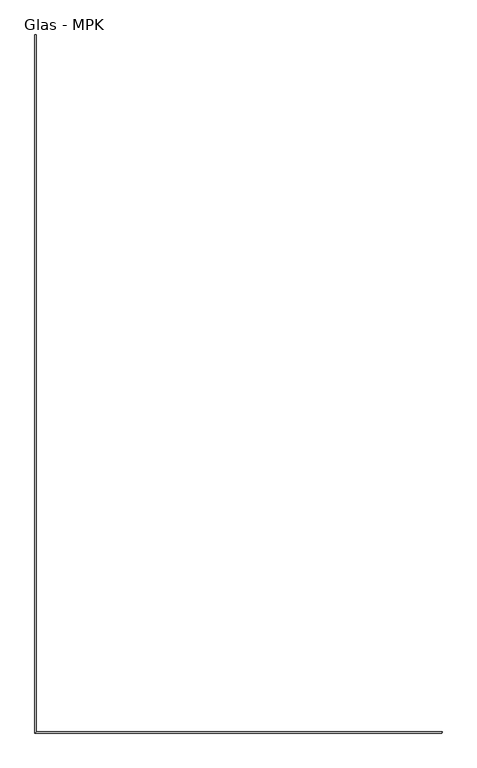
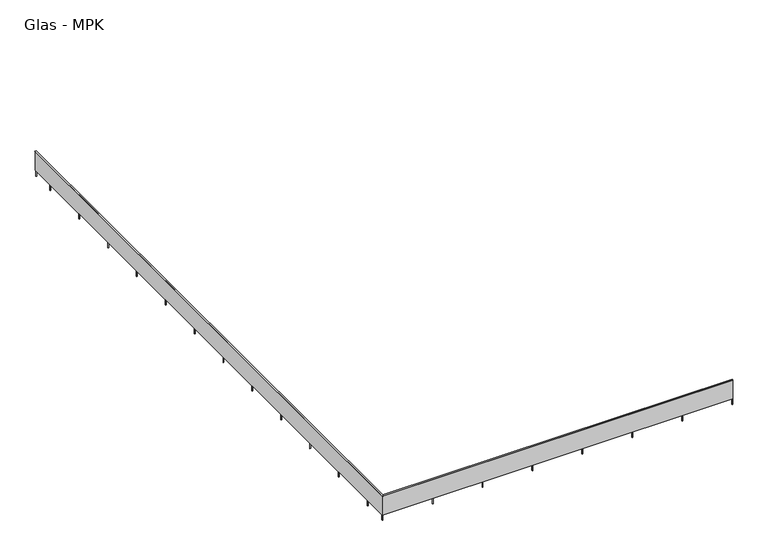
"""IFC4 building model written with IfcOpenShell, lengths in millimetres: railing geometry, Glas - MPK."""

from ifc_helpers import new_model, si_unit, frame, origin, place, context, project, spatial, polyline, outline, extrude, faceted_brep, source, transform, mapped, element, save


def glas_mpk_99f97afc(model_context):
    return source(origin(), model_context, "Body", "SolidModel", [
        faceted_brep([(22257.9971367, 15998.757723, 3843.2628643), (22207.9971367, 15998.757723, 3843.2628643), (22207.9971367, 15998.757723, 3856.7371357), (22257.9971367, 15998.757723, 3856.7371357), (36243.4971367, -8011.242277, 3843.2628643), (36243.4971367, -8011.242277, 3856.7371357), (36243.4971367, -8061.242277, 3856.7371357), (36243.4971367, -8061.242277, 3843.2628643), (22257.9971367, -8011.242277, 3843.2628643), (22207.9971367, -8061.242277, 3843.2628643), (22207.9971367, -8061.242277, 3856.7371357), (22257.9971367, -8011.242277, 3856.7371357)], [[[0, 1, 2, 3]], [[4, 5, 6, 7]], [[1, 0, 8, 9]], [[2, 1, 9, 10]], [[3, 2, 10, 11]], [[0, 3, 11, 8]], [[9, 8, 4, 7]], [[10, 9, 7, 6]], [[11, 10, 6, 5]], [[8, 11, 5, 4]]]),
        faceted_brep([(22217.9971367, 15998.757723, 3842.8769824), (22232.1892606, 15998.757723, 3842.8769824), (22232.1892606, 15998.757723, 3042.8769824), (22217.9971367, 15998.757723, 3042.8769824), (22217.9971367, -8051.242277, 3842.8769824), (22232.1892606, -8037.0501531, 3842.8769824), (22232.1892606, -8037.0501531, 3042.8769824), (22217.9971367, -8051.242277, 3042.8769824), (36243.4971367, -8051.242277, 3842.8769824), (36243.4971367, -8051.242277, 3042.8769824), (36243.4971367, -8037.0501531, 3042.8769824), (36243.4971367, -8037.0501531, 3842.8769824)], [[[0, 1, 2, 3]], [[1, 0, 4, 5]], [[2, 1, 5, 6]], [[3, 2, 6, 7]], [[0, 3, 7, 4]], [[8, 9, 10, 11]], [[5, 4, 8, 11]], [[6, 5, 11, 10]], [[7, 6, 10, 9]], [[4, 7, 9, 8]]]),
        extrude(outline(polyline([(34236.9971367, -8036.242277), (34236.9971367, -8011.242277), (34261.9971367, -8011.242277), (34261.9971367, -8036.242277), (34236.9971367, -8036.242277)])), frame((0.0, 0.0, 2800.0), z_axis=(0.0, 0.0, 1.0), x_axis=(1.0, 0.0, 0.0)), (0.0, 0.0, 1.0), 1043.2628643),
        extrude(outline(polyline([(32236.9971367, -8036.242277), (32236.9971367, -8011.242277), (32261.9971367, -8011.242277), (32261.9971367, -8036.242277), (32236.9971367, -8036.242277)])), frame((0.0, 0.0, 2800.0), z_axis=(0.0, 0.0, 1.0), x_axis=(1.0, 0.0, 0.0)), (0.0, 0.0, 1.0), 1043.2628643),
        extrude(outline(polyline([(30236.9971367, -8036.242277), (30236.9971367, -8011.242277), (30261.9971367, -8011.242277), (30261.9971367, -8036.242277), (30236.9971367, -8036.242277)])), frame((0.0, 0.0, 2800.0), z_axis=(0.0, 0.0, 1.0), x_axis=(1.0, 0.0, 0.0)), (0.0, 0.0, 1.0), 1043.2628643),
        extrude(outline(polyline([(28236.9971367, -8036.242277), (28236.9971367, -8011.242277), (28261.9971367, -8011.242277), (28261.9971367, -8036.242277), (28236.9971367, -8036.242277)])), frame((0.0, 0.0, 2800.0), z_axis=(0.0, 0.0, 1.0), x_axis=(1.0, 0.0, 0.0)), (0.0, 0.0, 1.0), 1043.2628643),
        extrude(outline(polyline([(26236.9971367, -8036.242277), (26236.9971367, -8011.242277), (26261.9971367, -8011.242277), (26261.9971367, -8036.242277), (26236.9971367, -8036.242277)])), frame((0.0, 0.0, 2800.0), z_axis=(0.0, 0.0, 1.0), x_axis=(1.0, 0.0, 0.0)), (0.0, 0.0, 1.0), 1043.2628643),
        extrude(outline(polyline([(24236.9971367, -8036.242277), (24236.9971367, -8011.242277), (24261.9971367, -8011.242277), (24261.9971367, -8036.242277), (24236.9971367, -8036.242277)])), frame((0.0, 0.0, 2800.0), z_axis=(0.0, 0.0, 1.0), x_axis=(1.0, 0.0, 0.0)), (0.0, 0.0, 1.0), 1043.2628643),
        extrude(outline(polyline([(22232.9971367, -6994.992277), (22257.9971367, -6994.992277), (22257.9971367, -7019.992277), (22232.9971367, -7019.992277), (22232.9971367, -6994.992277)])), frame((0.0, 0.0, 2800.0), z_axis=(0.0, 0.0, 1.0), x_axis=(1.0, 0.0, 0.0)), (0.0, 0.0, 1.0), 1043.2628643),
        extrude(outline(polyline([(22232.9971367, -4994.992277), (22257.9971367, -4994.992277), (22257.9971367, -5019.992277), (22232.9971367, -5019.992277), (22232.9971367, -4994.992277)])), frame((0.0, 0.0, 2800.0), z_axis=(0.0, 0.0, 1.0), x_axis=(1.0, 0.0, 0.0)), (0.0, 0.0, 1.0), 1043.2628643),
        extrude(outline(polyline([(22232.9971367, -2994.992277), (22257.9971367, -2994.992277), (22257.9971367, -3019.992277), (22232.9971367, -3019.992277), (22232.9971367, -2994.992277)])), frame((0.0, 0.0, 2800.0), z_axis=(0.0, 0.0, 1.0), x_axis=(1.0, 0.0, 0.0)), (0.0, 0.0, 1.0), 1043.2628643),
        extrude(outline(polyline([(22232.9971367, -994.992277), (22257.9971367, -994.992277), (22257.9971367, -1019.992277), (22232.9971367, -1019.992277), (22232.9971367, -994.992277)])), frame((0.0, 0.0, 2800.0), z_axis=(0.0, 0.0, 1.0), x_axis=(1.0, 0.0, 0.0)), (0.0, 0.0, 1.0), 1043.2628643),
        extrude(outline(polyline([(22232.9971367, 1005.007723), (22257.9971367, 1005.007723), (22257.9971367, 980.007723), (22232.9971367, 980.007723), (22232.9971367, 1005.007723)])), frame((0.0, 0.0, 2800.0), z_axis=(0.0, 0.0, 1.0), x_axis=(1.0, 0.0, 0.0)), (0.0, 0.0, 1.0), 1043.2628643),
        extrude(outline(polyline([(22232.9971367, 3005.007723), (22257.9971367, 3005.007723), (22257.9971367, 2980.007723), (22232.9971367, 2980.007723), (22232.9971367, 3005.007723)])), frame((0.0, 0.0, 2800.0), z_axis=(0.0, 0.0, 1.0), x_axis=(1.0, 0.0, 0.0)), (0.0, 0.0, 1.0), 1043.2628643),
        extrude(outline(polyline([(22232.9971367, 5005.007723), (22257.9971367, 5005.007723), (22257.9971367, 4980.007723), (22232.9971367, 4980.007723), (22232.9971367, 5005.007723)])), frame((0.0, 0.0, 2800.0), z_axis=(0.0, 0.0, 1.0), x_axis=(1.0, 0.0, 0.0)), (0.0, 0.0, 1.0), 1043.2628643),
        extrude(outline(polyline([(22232.9971367, 7005.007723), (22257.9971367, 7005.007723), (22257.9971367, 6980.007723), (22232.9971367, 6980.007723), (22232.9971367, 7005.007723)])), frame((0.0, 0.0, 2800.0), z_axis=(0.0, 0.0, 1.0), x_axis=(1.0, 0.0, 0.0)), (0.0, 0.0, 1.0), 1043.2628643),
        extrude(outline(polyline([(22232.9971367, 9005.007723), (22257.9971367, 9005.007723), (22257.9971367, 8980.007723), (22232.9971367, 8980.007723), (22232.9971367, 9005.007723)])), frame((0.0, 0.0, 2800.0), z_axis=(0.0, 0.0, 1.0), x_axis=(1.0, 0.0, 0.0)), (0.0, 0.0, 1.0), 1043.2628643),
        extrude(outline(polyline([(22232.9971367, 11005.007723), (22257.9971367, 11005.007723), (22257.9971367, 10980.007723), (22232.9971367, 10980.007723), (22232.9971367, 11005.007723)])), frame((0.0, 0.0, 2800.0), z_axis=(0.0, 0.0, 1.0), x_axis=(1.0, 0.0, 0.0)), (0.0, 0.0, 1.0), 1043.2628643),
        extrude(outline(polyline([(22232.9971367, 13005.007723), (22257.9971367, 13005.007723), (22257.9971367, 12980.007723), (22232.9971367, 12980.007723), (22232.9971367, 13005.007723)])), frame((0.0, 0.0, 2800.0), z_axis=(0.0, 0.0, 1.0), x_axis=(1.0, 0.0, 0.0)), (0.0, 0.0, 1.0), 1043.2628643),
        extrude(outline(polyline([(22232.9971367, 15005.007723), (22257.9971367, 15005.007723), (22257.9971367, 14980.007723), (22232.9971367, 14980.007723), (22232.9971367, 15005.007723)])), frame((0.0, 0.0, 2800.0), z_axis=(0.0, 0.0, 1.0), x_axis=(1.0, 0.0, 0.0)), (0.0, 0.0, 1.0), 1043.2628643),
        extrude(outline(polyline([(22232.9971367, -8001.242277), (22257.9971367, -8001.242277), (22257.9971367, -8026.242277), (22232.9971367, -8026.242277), (22232.9971367, -8001.242277)])), frame((0.0, 0.0, 2800.0), z_axis=(0.0, 0.0, 1.0), x_axis=(1.0, 0.0, 0.0)), (0.0, 0.0, 1.0), 1043.2628643),
        extrude(outline(polyline([(36230.9971367, -8036.242277), (36230.9971367, -8011.242277), (36255.9971367, -8011.242277), (36255.9971367, -8036.242277), (36230.9971367, -8036.242277)])), frame((0.0, 0.0, 2800.0), z_axis=(0.0, 0.0, 1.0), x_axis=(1.0, 0.0, 0.0)), (0.0, 0.0, 1.0), 1043.2628643),
        extrude(outline(polyline([(22232.9971367, 15998.757723), (22257.9971367, 15998.757723), (22257.9971367, 15973.757723), (22232.9971367, 15973.757723), (22232.9971367, 15998.757723)])), frame((0.0, 0.0, 2800.0), z_axis=(0.0, 0.0, 1.0), x_axis=(1.0, 0.0, 0.0)), (0.0, 0.0, 1.0), 1043.2628643),
    ])


if __name__ == "__main__":
    model = new_model("IFC4")
    model_context = context("Model", 3, world=origin())
    ifc_project = project(units=[si_unit("LENGTHUNIT", "METRE", prefix="MILLI")], contexts=[model_context])
    site = spatial("IfcSite", under=ifc_project)
    building = spatial("IfcBuilding", under=site)
    placement = place(None, origin())
    glas_mpk_shape = glas_mpk_99f97afc(model_context)
    element("IfcRailing", 1, ObjectType="Glas - MPK", at=placement, inside=building, context=model_context, shape_type="MappedRepresentation", body=[
        mapped(glas_mpk_shape, transform((0.0, 0.0, 0.0), x_axis=(1.0, 0.0, 0.0), y_axis=(0.0, 1.0, 0.0), z_axis=(0.0, 0.0, 1.0))),
    ])
    save(model, "model.ifc")

# Revit data of these elements
# Element 1 (IfcRailing, "Glas - MPK")
#   Materials on its faces: "Metal - Aluminum", "Window - Glass"
# Materials
#   "Metal - Aluminum": class "Unassigned", colour RGB 247 247 247, transparency 0, Comments = "Rendering appearance not upgraded "
#   "Window - Glass": class "Glas", colour RGB 128 128 255, transparency 0.75
